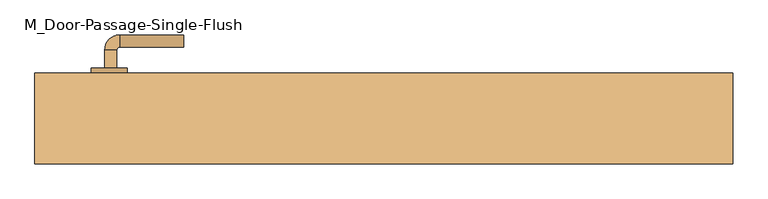
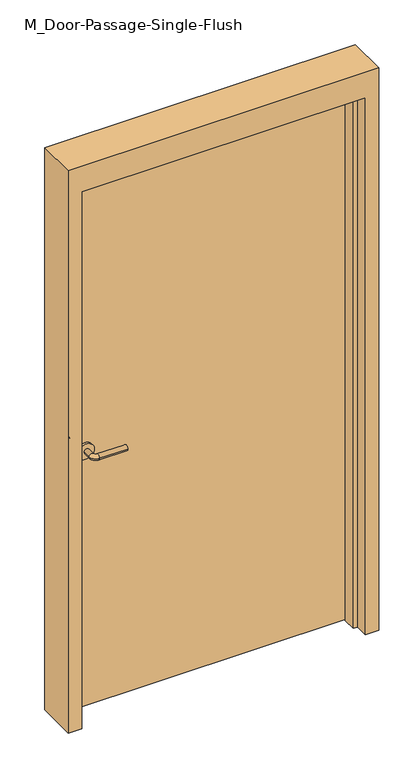
"""IFC4 building model written with IfcOpenShell, lengths in millimetres: door geometry, M_Door-Passage-Single-Flush : H_DR_AMD_Single Door_Int_Steel_1050x2100."""

from ifc_helpers import new_model, si_unit, point, frame, frame_2d, origin, origin_with_axes, place, context, project, spatial, polyline, circle_curve, ellipse_curve, trimmed, segment, composite_curve, outline, extrude, faceted_brep, source, transform, mapped, element, save
from ifc_brep_helpers import plane_surface, cylinder_surface, revolved_surface, advanced_brep


def m_door_passage_single_flush_8c4eadbe(model_context):
    return source(origin(), model_context, "Body", "SolidModel", [
        advanced_brep(
        [(-459.990625, 35.35, 1000.0), (-439.990625, 35.35, 1000.0), (-439.990625, 5.35, 1000.0), (-459.990625, 5.35, 1000.0), (-434.990625, 0.35, 1000.0), (-434.990625, -19.65, 1000.0), (-329.990625, -19.65, 1000.0), (-329.990625, 0.35, 1000.0)],
        [
            (0, 1, circle_curve(frame((-449.990625, 35.35, 1000.0), z_axis=(0.0, 1.0, 0.0), x_axis=(1.0, 0.0, 0.0)), 10.0)),
            (1, 0, circle_curve(frame((-449.990625, 35.35, 1000.0), z_axis=(0.0, 1.0, 0.0), x_axis=(1.0, 0.0, 0.0)), 10.0)),
            (1, 2),
            (2, 3, circle_curve(frame((-449.990625, 5.35, 1000.0), z_axis=(0.0, 1.0, 0.0), x_axis=(1.0, 0.0, 0.0)), 10.0)),
            (3, 0),
            (3, 2, circle_curve(frame((-449.990625, 5.35, 1000.0), z_axis=(0.0, 1.0, 0.0), x_axis=(1.0, 0.0, 0.0)), 10.0)),
            (4, 5, circle_curve(frame((-434.990625, -9.65, 1000.0), z_axis=(-1.0, 0.0, 0.0), x_axis=(0.0, 1.0, 0.0)), 10.0)),
            (5, 3, circle_curve(frame((-434.990625, 5.35, 1000.0), z_axis=(0.0, 0.0, -1.0), x_axis=(-1.0, 0.0, 0.0)), 25.0)),
            (2, 4, circle_curve(frame((-434.990625, 5.35, 1000.0), z_axis=(0.0, 0.0, 1.0), x_axis=(-1.0, 0.0, 0.0)), 5.0)),
            (5, 4, circle_curve(frame((-434.990625, -9.65, 1000.0), z_axis=(-1.0, 0.0, 0.0), x_axis=(0.0, 1.0, 0.0)), 10.0)),
            (6, 7, circle_curve(frame((-329.990625, -9.65, 1000.0), z_axis=(1.0, 0.0, 0.0), x_axis=(0.0, 1.0, 0.0)), 10.0)),
            (7, 6, circle_curve(frame((-329.990625, -9.65, 1000.0), z_axis=(1.0, 0.0, 0.0), x_axis=(0.0, 1.0, 0.0)), 10.0)),
            (4, 7),
            (6, 5),
        ],
        [
            plane_surface(frame((-449.990625, 35.35, 1000.0), z_axis=(0.0, 1.0, 0.0), x_axis=(0.0, 0.0, 1.0))),
            cylinder_surface(frame((-449.990625, 35.35, 1000.0), z_axis=(0.0, 1.0, 0.0), x_axis=(1.0, 0.0, 0.0)), 10.0),
            revolved_surface(trimmed(ellipse_curve(frame((-449.990625, 5.35, 1000.0), z_axis=(0.0, -1.0, 0.0), x_axis=(1.0, 0.0, 0.0)), 10.0, 10.0), [point((-459.990625, 5.35, 1000.0))], [point((-439.990625, 5.35, 1000.0))], True, "CARTESIAN"), (-434.990625, 5.35, 1000.0), (0.0, 0.0, -1.0)),
            revolved_surface(trimmed(ellipse_curve(frame((-449.990625, 5.35, 1000.0), z_axis=(0.0, -1.0, 0.0), x_axis=(1.0, 0.0, 0.0)), 10.0, 10.0), [point((-439.990625, 5.35, 1000.0))], [point((-459.990625, 5.35, 1000.0))], True, "CARTESIAN"), (-434.990625, 5.35, 1000.0), (0.0, 0.0, -1.0)),
            plane_surface(frame((-329.990625, -9.65, 1000.0), z_axis=(1.0, 0.0, 0.0), x_axis=(0.0, 0.0, 1.0))),
            cylinder_surface(frame((-434.990625, -9.65, 1000.0), z_axis=(-1.0, 0.0, 0.0), x_axis=(0.0, 1.0, 0.0)), 10.0),
        ],
        [
            (0, [[1, 2]]),
            (1, [[3, 4, 5, -2]]),
            (1, [[-5, 6, -3, -1]]),
            (2, [[7, 8, -4, 9]]),
            (3, [[10, -9, -6, -8]]),
            (4, [[11, 12]]),
            (5, [[13, -11, 14, -7]]),
            (5, [[-14, -12, -13, -10]]),
        ],
    ),
        extrude(outline(composite_curve([segment(trimmed(circle_curve(frame_2d((1000.0, -452.490625)), 30.0), [point((1000.0, -482.490625))], [point((1000.0, -422.490625))], False, "CARTESIAN"), True, "CONTINUOUS"), segment(trimmed(circle_curve(frame_2d((1000.0, -452.490625)), 30.0), [point((1000.0, -422.490625))], [point((1000.0, -482.490625))], False, "CARTESIAN"), True, "CONTINUOUS")], self_intersect=False)), frame((0.0, 35.35, 0.0), z_axis=(0.0, 1.0, 0.0), x_axis=(0.0, 0.0, 1.0)), (0.0, 0.0, 1.0), 8.0),
        advanced_brep(
        [(-459.990625, 96.35, 1000.0), (-439.990625, 96.35, 1000.0), (-459.990625, 126.35, 1000.0), (-439.990625, 126.35, 1000.0), (-434.990625, 131.35, 1000.0), (-434.990625, 151.35, 1000.0), (-329.990625, 151.35, 1000.0), (-329.990625, 131.35, 1000.0)],
        [
            (0, 1, circle_curve(frame((-449.990625, 96.35, 1000.0), z_axis=(0.0, -1.0, 0.0), x_axis=(1.0, 0.0, 0.0)), 10.0)),
            (1, 0, circle_curve(frame((-449.990625, 96.35, 1000.0), z_axis=(0.0, -1.0, 0.0), x_axis=(1.0, 0.0, 0.0)), 10.0)),
            (0, 2),
            (2, 3, circle_curve(frame((-449.990625, 126.35, 1000.0), z_axis=(0.0, -1.0, 0.0), x_axis=(1.0, 0.0, 0.0)), 10.0)),
            (3, 1),
            (3, 2, circle_curve(frame((-449.990625, 126.35, 1000.0), z_axis=(0.0, -1.0, 0.0), x_axis=(1.0, 0.0, 0.0)), 10.0)),
            (4, 3, circle_curve(frame((-434.990625, 126.35, 1000.0), z_axis=(0.0, 0.0, 1.0), x_axis=(-1.0, 0.0, 0.0)), 5.0)),
            (2, 5, circle_curve(frame((-434.990625, 126.35, 1000.0), z_axis=(0.0, 0.0, -1.0), x_axis=(-1.0, 0.0, 0.0)), 25.0)),
            (5, 4, circle_curve(frame((-434.990625, 141.35, 1000.0), z_axis=(-1.0, 0.0, 0.0), x_axis=(0.0, -1.0, 0.0)), 10.0)),
            (4, 5, circle_curve(frame((-434.990625, 141.35, 1000.0), z_axis=(-1.0, 0.0, 0.0), x_axis=(0.0, -1.0, 0.0)), 10.0)),
            (6, 7, circle_curve(frame((-329.990625, 141.35, 1000.0), z_axis=(1.0, 0.0, 0.0), x_axis=(0.0, -1.0, 0.0)), 10.0)),
            (7, 6, circle_curve(frame((-329.990625, 141.35, 1000.0), z_axis=(1.0, 0.0, 0.0), x_axis=(0.0, -1.0, 0.0)), 10.0)),
            (5, 6),
            (7, 4),
        ],
        [
            plane_surface(frame((-449.990625, 96.35, 1000.0), z_axis=(0.0, -1.0, 0.0), x_axis=(0.0, 0.0, 1.0))),
            cylinder_surface(frame((-449.990625, 96.35, 1000.0), z_axis=(0.0, -1.0, 0.0), x_axis=(1.0, 0.0, 0.0)), 10.0),
            revolved_surface(trimmed(ellipse_curve(frame((-449.990625, 126.35, 1000.0), z_axis=(0.0, -1.0, 0.0), x_axis=(1.0, 0.0, 0.0)), 10.0, 10.0), [point((-459.990625, 126.35, 1000.0))], [point((-439.990625, 126.35, 1000.0))], True, "CARTESIAN"), (-434.990625, 126.35, 1000.0), (0.0, 0.0, -1.0)),
            revolved_surface(trimmed(ellipse_curve(frame((-449.990625, 126.35, 1000.0), z_axis=(0.0, -1.0, 0.0), x_axis=(1.0, 0.0, 0.0)), 10.0, 10.0), [point((-439.990625, 126.35, 1000.0))], [point((-459.990625, 126.35, 1000.0))], True, "CARTESIAN"), (-434.990625, 126.35, 1000.0), (0.0, 0.0, -1.0)),
            plane_surface(frame((-329.990625, 141.35, 1000.0), z_axis=(1.0, 0.0, 0.0), x_axis=(0.0, 0.0, 1.0))),
            cylinder_surface(frame((-434.990625, 141.35, 1000.0), z_axis=(-1.0, 0.0, 0.0), x_axis=(0.0, -1.0, 0.0)), 10.0),
        ],
        [
            (0, [[1, 2]]),
            (1, [[-1, 3, 4, 5]]),
            (1, [[-2, -5, 6, -3]]),
            (2, [[7, -4, 8, 9]]),
            (3, [[-8, -6, -7, 10]]),
            (4, [[11, 12]]),
            (5, [[-9, 13, -12, 14]]),
            (5, [[-10, -14, -11, -13]]),
        ],
    ),
        extrude(outline(composite_curve([segment(trimmed(circle_curve(frame_2d((1000.0, -452.490625)), 30.0), [point((1000.0, -482.490625))], [point((1000.0, -422.490625))], False, "CARTESIAN"), True, "CONTINUOUS"), segment(trimmed(circle_curve(frame_2d((1000.0, -452.490625)), 30.0), [point((1000.0, -422.490625))], [point((1000.0, -482.490625))], False, "CARTESIAN"), True, "CONTINUOUS")], self_intersect=False)), frame((0.0, 88.35, 0.0), z_axis=(0.0, 1.0, 0.0), x_axis=(0.0, 0.0, 1.0)), (0.0, 0.0, 1.0), 8.0),
        faceted_brep([(525.0, 38.5875, 0.0), (525.0, 88.35, 0.0), (575.0, 88.35, 0.0), (575.0, -61.65, 0.0), (525.0, -61.65, 0.0), (525.0, -12.4375, 0.0), (509.125, -12.4375, 0.0), (509.125, 38.5875, 0.0), (525.0, 38.5875, 2100.0), (525.0, 88.35, 2100.0), (-525.0, 88.35, 2100.0), (-525.0, 88.35, 0.0), (-575.0, 88.35, 0.0), (-575.0, 88.35, 2200.0), (575.0, 88.35, 2200.0), (575.0, -61.65, 2200.0), (-575.0, -61.65, 2200.0), (-575.0, -61.65, 0.0), (-525.0, -61.65, 0.0), (-525.0, -61.65, 2100.0), (525.0, -61.65, 2100.0), (525.0, -12.4375, 2100.0), (-525.0, -12.4375, 2100.0), (-525.0, -12.4375, 0.0), (-509.125, -12.4375, 0.0), (-509.125, -12.4375, 2084.125), (509.125, -12.4375, 2084.125), (509.125, 38.5875, 2084.125), (-509.125, 38.5875, 2084.125), (-509.125, 38.5875, 0.0), (-525.0, 38.5875, 0.0), (-525.0, 38.5875, 2100.0)], [[[0, 1, 2, 3, 4, 5, 6, 7]], [[1, 0, 8, 9]], [[2, 1, 9, 10, 11, 12, 13, 14]], [[3, 2, 14, 15]], [[4, 3, 15, 16, 17, 18, 19, 20]], [[5, 4, 20, 21]], [[6, 5, 21, 22, 23, 24, 25, 26]], [[7, 6, 26, 27]], [[0, 7, 27, 28, 29, 30, 31, 8]], [[9, 8, 31, 10]], [[20, 19, 22, 21]], [[26, 25, 28, 27]], [[12, 11, 30, 29, 24, 23, 18, 17]], [[11, 10, 31, 30]], [[13, 12, 17, 16]], [[19, 18, 23, 22]], [[25, 24, 29, 28]], [[15, 14, 13, 16]]]),
        extrude(outline(polyline([(525.0, 43.35), (-525.0, 43.35), (-525.0, 88.35), (525.0, 88.35), (525.0, 43.35)])), origin_with_axes(), (0.0, 0.0, 1.0), 2100.0),
    ])


if __name__ == "__main__":
    model = new_model("IFC4")
    model_context = context("Model", 3, world=origin())
    ifc_project = project(units=[si_unit("LENGTHUNIT", "METRE", prefix="MILLI")], contexts=[model_context])
    site = spatial("IfcSite", under=ifc_project)
    building = spatial("IfcBuilding", under=site)
    placement = place(None, origin())
    m_door_passage_single_flush_shape = m_door_passage_single_flush_8c4eadbe(model_context)
    element("IfcDoor", 1, ObjectType="M_Door-Passage-Single-Flush : H_DR_AMD_Single Door_Int_Steel_1050x2100", at=placement, inside=building, context=model_context, shape_type="MappedRepresentation", body=[
        mapped(m_door_passage_single_flush_shape, transform((0.0, 0.0, 0.0), x_axis=(1.0, 0.0, 0.0), y_axis=(0.0, 1.0, 0.0), z_axis=(0.0, 0.0, 1.0))),
    ])
    save(model, "model.ifc")

# Revit data of these elements
# Type "M_Door-Passage-Single-Flush : H_DR_AMD_Single Door_Int_Steel_1050x2100"
#   Type Mark = "SD"
#   Assembly Code = "B2030200"
#   Analytic Construction = "Wooden"
#   Thickness = 0.0450 m
#   Thermal Resistance (R) = 0.455703 (m²·K)/W
#   Swing Angle [instance default] = 90.00°
#   Strike Height = 1.0000 m
#   Rough Width [instance default] = 1.1500 m
#   Rough Height [instance default] = 2.2000 m
#   MF Opening Height [instance default] = 0.1000 m
#   MF Opening Width [instance default] = 0.1000 m
#   Inset Calculate [instance default] = 0.1050 m
#   Masonry Inset [instance default] = 0.0250 m
#   Height = 2.1000 m
#   Width = 1.0500 m
#   Heat Transfer Coefficient (U) = 2.19465 W/(m²·K)
#   Masonry Frame Depth = 0.1500 m
#   Masonry Frame [instance default] = yes
#   Dry Wall Frame [instance default] = no
#   Panel Material = Wood - Birch
#   Frame Material = Metal - Paint Finish - Grey
#   Door Handle Material = Aluminum
#   Visual Light Transmittance = 0
#   Solar Heat Gain Coefficient = 0
#   Wall Closure = (empty or 0)
#   Function = (empty or 0)
# Element 1 (IfcDoor, "M_Door-Passage-Single-Flush : H_DR_AMD_Single Door_Int_Steel_1050x2100")
#   Materials on its faces: "Aluminum", "Metal - Paint Finish - Grey", "Wood - Birch"
# Materials
#   "Wood - Birch": class "Wood", colour RGB 166 116 52, transparency 0, Cost = 0
#   "Metal - Paint Finish - Grey": class "Paint", colour RGB 104 104 104, transparency 0, Cost = 0
#   "Aluminum": class "Metal", colour RGB 244 244 244, transparency 0, Description = "Aluminum 6061", Cost = 0
